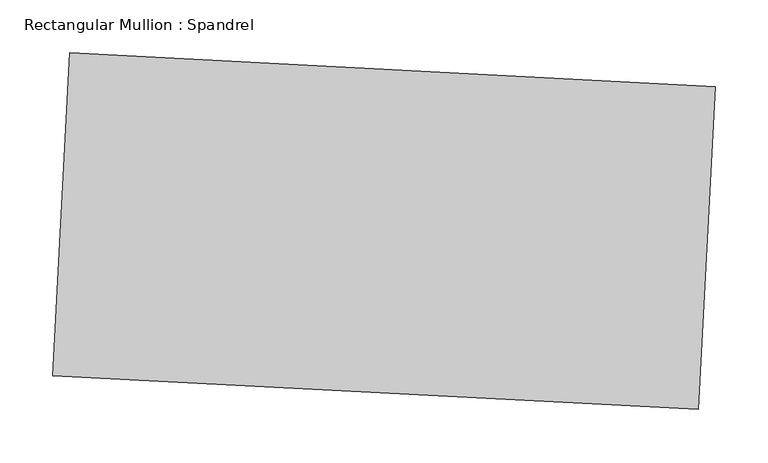
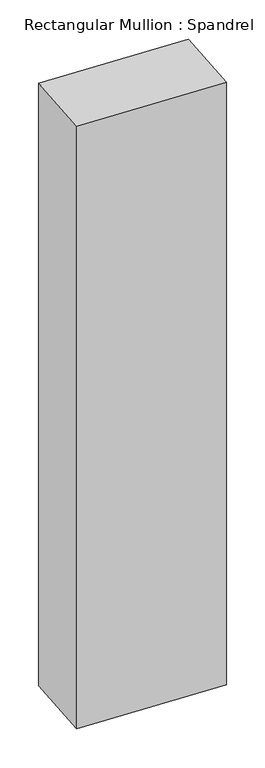
"""IFC4 building model written with IfcOpenShell, lengths in millimetres: member geometry, Rectangular Mullion : Spandrel."""

from ifc_helpers import new_model, si_unit, frame, origin, place, context, project, spatial, polyline, outline, extrude, source, transform, mapped, element, save


def rectangular_mullion_spandrel_2df0ba9b(model_context):
    return source(origin(), model_context, "Body", "SweptSolid", [
        extrude(outline(polyline([(312.3582819, 136.2391416), (296.4062825, -168.1431406), (-312.3582819, -136.2391416), (-296.4062825, 168.1431406), (312.3582819, 136.2391416)])), frame((0.0, 0.0, -2667.6321869), z_axis=(0.0, 0.0, 1.0), x_axis=(1.0, 0.0, 0.0)), (0.0, 0.0, 1.0), 2667.6321869),
    ])


if __name__ == "__main__":
    model = new_model("IFC4")
    model_context = context("Model", 3, world=origin())
    ifc_project = project(units=[si_unit("LENGTHUNIT", "METRE", prefix="MILLI")], contexts=[model_context])
    site = spatial("IfcSite", under=ifc_project)
    building = spatial("IfcBuilding", under=site)
    placement = place(None, origin())
    rectangular_mullion_spandrel_shape = rectangular_mullion_spandrel_2df0ba9b(model_context)
    element("IfcMember", 1, ObjectType="Rectangular Mullion : Spandrel", at=placement, inside=building, context=model_context, shape_type="MappedRepresentation", body=[
        mapped(rectangular_mullion_spandrel_shape, transform((0.0, 0.0, 0.0), x_axis=(1.0, 0.0, 0.0), y_axis=(0.0, 1.0, 0.0), z_axis=(0.0, 0.0, 1.0))),
    ])
    save(model, "model.ifc")

# Revit data of these elements
# Type "Rectangular Mullion : Spandrel"
#   built-in parameter 1007304 = 1 (stored number, unit not read)
#   built-in parameter 1007301 = 1 (stored number, unit not read)
#   built-in parameter 1007300 = 1 (stored number, unit not read)
# Element 1 (IfcMember, "Rectangular Mullion : Spandrel")
#   Materials on its faces: "Aluminum"
# Materials
#   "Aluminum": class "Metal", colour RGB 247 247 247, transparency 0, Description = "Aluminum 6061", Cost = 0
